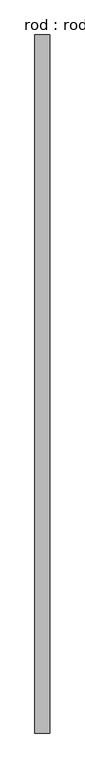
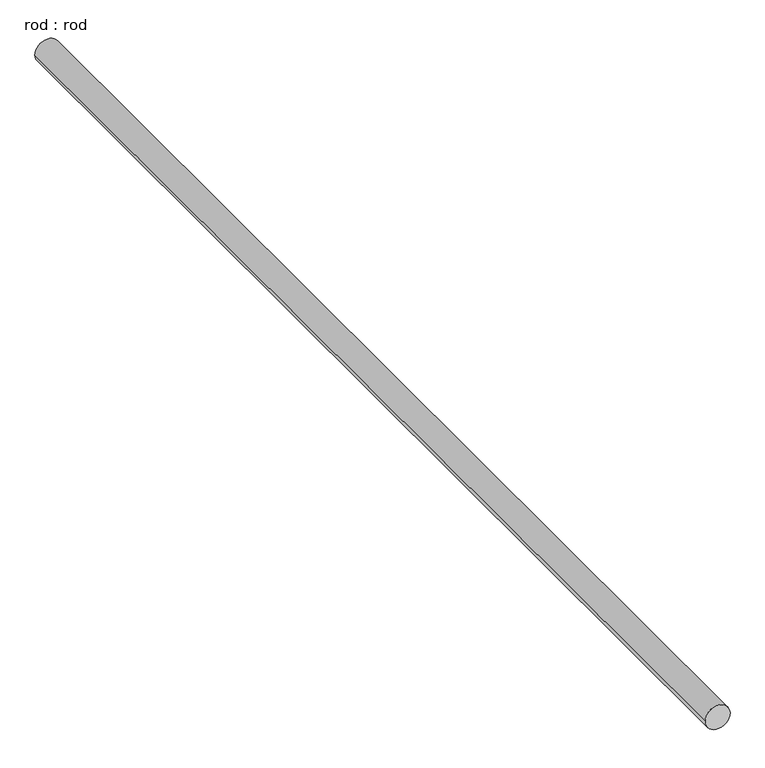
"""IFC4 building model written with IfcOpenShell, lengths in millimetres: proxy geometry, rod : rod."""

import ifcopenshell
import ifcopenshell.guid

model = None  # the IFC model being written
_history = None  # IfcOwnerHistory: only IFC2X3 demands one
_inside = {}  # id of a spatial element -> (the spatial element, [elements in it])
_under = {}  # id of a project, library or spatial element -> (it, [spatial elements below it])
_declared = {}  # id of a project -> (the project, [libraries it declares])
_typed = {}  # id of a type object -> (the type object, [elements of that type])
_made_of = {}  # id of a material, layer set ... -> (it, [elements and type objects made of it])


def new_model(schema):
    """Start an empty IFC model of exactly this schema.

    Asked for "IFC4X3", IfcOpenShell would pick the latest addendum, in which some entities
    have other attributes; the version numbers below select the first issue.
    IFC2X3 requires an IfcOwnerHistory on every rooted entity: one is made here for all.
    """
    global model, _history
    if schema == "IFC4X3":
        model = ifcopenshell.file(schema_version=(4, 3, 0, 0))
    else:
        model = ifcopenshell.file(schema=schema)
    _inside.clear()
    _under.clear()
    _declared.clear()
    _typed.clear()
    _made_of.clear()
    _history = None
    if model.schema == "IFC2X3":
        org = make("IfcOrganization", Name="unknown")
        user = make(
            "IfcPersonAndOrganization",
            ThePerson=make("IfcPerson", FamilyName="unknown"),
            TheOrganization=org,
        )
        app = make(
            "IfcApplication",
            ApplicationDeveloper=org,
            Version="unknown",
            ApplicationFullName="unknown",
            ApplicationIdentifier="unknown",
        )
        _history = make(
            "IfcOwnerHistory",
            OwningUser=user,
            OwningApplication=app,
            ChangeAction="ADDED",
            CreationDate=0,
        )
    return model


def make(cls, **values):
    """One entity of the class cls with the attributes given. An attribute that is None is left unset."""
    return model.create_entity(
        cls, **{name: value for name, value in values.items() if value is not None}
    )


def rooted(cls, **values):
    """An entity with a GlobalId (a new one), such as an element, a storey or a relation."""
    return make(cls, GlobalId=ifcopenshell.guid.new(), OwnerHistory=_history, **values)


def si_unit(unit_type, name, prefix=None):
    """IfcSIUnit, for example si_unit("LENGTHUNIT", "METRE", prefix="MILLI")."""
    return make("IfcSIUnit", UnitType=unit_type, Prefix=prefix, Name=name)


def assignment(units):
    """IfcUnitAssignment: the units of a project."""
    return None if units is None else make("IfcUnitAssignment", Units=units)


def point(xyz):
    """IfcCartesianPoint."""
    return None if xyz is None else make("IfcCartesianPoint", Coordinates=xyz)


def direction(xyz):
    """IfcDirection."""
    return None if xyz is None else make("IfcDirection", DirectionRatios=xyz)


def frame(location, z_axis=None, x_axis=None):
    """IfcAxis2Placement3D, a coordinate frame: its origin and axes. An axis left out is left unset."""
    return make(
        "IfcAxis2Placement3D",
        Location=point(location),
        Axis=direction(z_axis),
        RefDirection=direction(x_axis),
    )


def frame_2d(location, x_axis=None):
    """IfcAxis2Placement2D, a coordinate frame in the plane: its origin and x axis."""
    return make(
        "IfcAxis2Placement2D", Location=point(location), RefDirection=direction(x_axis)
    )


def origin():
    """The frame at (0, 0, 0) with its axes left unset."""
    return frame((0.0, 0.0, 0.0))


def place(relative_to, where):
    """IfcLocalPlacement: puts the frame where relative to a parent placement (None: the world)."""
    return make(
        "IfcLocalPlacement", PlacementRelTo=relative_to, RelativePlacement=where
    )


def context(
    kind, dimensions, precision=None, world=None, true_north=None, identifier=None
):
    """IfcGeometricRepresentationContext, for example the 3D "Model" context."""
    return make(
        "IfcGeometricRepresentationContext",
        ContextIdentifier=identifier,
        ContextType=kind,
        CoordinateSpaceDimension=dimensions,
        Precision=precision,
        WorldCoordinateSystem=world,
        TrueNorth=true_north,
    )


def project(units=None, contexts=None):
    """IfcProject with its units and contexts."""
    return rooted(
        "IfcProject",
        Name="project",
        RepresentationContexts=contexts,
        UnitsInContext=assignment(units),
    )


def spatial(cls, under=None, at=None, **own):
    """A site, building, storey or space (cls), placed at a placement, below another one or the project."""
    s = rooted(cls, ObjectPlacement=at, **own)
    if under is not None:
        _under.setdefault(under.id(), (under, []))[1].append(s)
    return s


def circle_curve(where, radius):
    """IfcCircle in the frame where."""
    return make("IfcCircle", Position=where, Radius=radius)


def trimmed(basis, trim1, trim2, sense, master):
    """IfcTrimmedCurve: the piece of a basis curve between two trims."""
    return make(
        "IfcTrimmedCurve",
        BasisCurve=basis,
        Trim1=trim1,
        Trim2=trim2,
        SenseAgreement=sense,
        MasterRepresentation=master,
    )


def segment(curve, same_sense, transition):
    """IfcCompositeCurveSegment."""
    return make(
        "IfcCompositeCurveSegment",
        Transition=transition,
        SameSense=same_sense,
        ParentCurve=curve,
    )


def composite_curve(segments, self_intersect=None):
    """IfcCompositeCurve: segments joined end to end."""
    return make("IfcCompositeCurve", Segments=segments, SelfIntersect=self_intersect)


def outline(outer, holes=None, kind="AREA"):
    """IfcArbitraryClosedProfileDef: a profile drawn as a closed curve; with holes, ...WithVoids."""
    if holes is None:
        return make("IfcArbitraryClosedProfileDef", ProfileType=kind, OuterCurve=outer)
    return make(
        "IfcArbitraryProfileDefWithVoids",
        ProfileType=kind,
        OuterCurve=outer,
        InnerCurves=holes,
    )


def extrude(swept, where, along, depth):
    """IfcExtrudedAreaSolid: the profile swept, set in the frame where, extruded along a direction by depth."""
    return make(
        "IfcExtrudedAreaSolid",
        SweptArea=swept,
        Position=where,
        ExtrudedDirection=direction(along),
        Depth=depth,
    )


def shape(context_of_items, identifier, shape_type, items):
    """IfcShapeRepresentation: the items that make up one representation, for example the "Body"."""
    return make(
        "IfcShapeRepresentation",
        ContextOfItems=context_of_items,
        RepresentationIdentifier=identifier,
        RepresentationType=shape_type,
        Items=items,
    )


def source(mapping_origin, context_of_items, identifier, shape_type, items):
    """IfcRepresentationMap: a shape defined once, which mapped items show again and again."""
    return make(
        "IfcRepresentationMap",
        MappingOrigin=mapping_origin,
        MappedRepresentation=shape(context_of_items, identifier, shape_type, items),
    )


def transform(
    local_origin,
    x_axis=None,
    y_axis=None,
    z_axis=None,
    scale=None,
    scale2=None,
    scale3=None,
    uniform=True,
):
    """IfcCartesianTransformationOperator3D, or its non-uniform kind. x_axis, y_axis, z_axis: its Axis1, 2, 3."""
    if uniform:
        return make(
            "IfcCartesianTransformationOperator3D",
            Axis1=direction(x_axis),
            Axis2=direction(y_axis),
            LocalOrigin=point(local_origin),
            Scale=scale,
            Axis3=direction(z_axis),
        )
    return make(
        "IfcCartesianTransformationOperator3DnonUniform",
        Axis1=direction(x_axis),
        Axis2=direction(y_axis),
        LocalOrigin=point(local_origin),
        Scale=scale,
        Axis3=direction(z_axis),
        Scale2=scale2,
        Scale3=scale3,
    )


def mapped(mapping_source, mapping_target):
    """IfcMappedItem: shows the shape of a source again, moved by a transform."""
    return make(
        "IfcMappedItem", MappingSource=mapping_source, MappingTarget=mapping_target
    )


def made_of(thing, what):
    """Note that an element or type object is made of a material, layer set ...; save() writes the relation."""
    if what is not None:
        _made_of.setdefault(what.id(), (what, []))[1].append(thing)
    return thing


def element(
    cls,
    number,
    at=None,
    inside=None,
    cuts=None,
    type_object=None,
    material=None,
    context=None,
    identifier="Body",
    shape_type=None,
    held_by="IfcProductDefinitionShape",
    body=None,
    shapes=None,
    **own,
):
    """One element of the class cls, such as IfcWall. Its Tag is "e" and its number.

    at: its placement. inside: the storey or other place that contains it. cuts: it is an
    opening in that element (IfcRelVoidsElement). A single representation is given by context,
    identifier, shape_type and body (its items); several are given by shapes. held_by: the class
    of the entity that holds the representations. save() writes the other relations.
    """
    e = rooted(cls, Tag="e%d" % number, ObjectPlacement=at, **own)
    if body is not None:
        shapes = [shape(context, identifier, shape_type, body)]
    if shapes is not None:
        e.Representation = make(held_by, Representations=shapes)
    if inside is not None:
        _inside.setdefault(inside.id(), (inside, []))[1].append(e)
    if cuts is not None:
        rooted(
            "IfcRelVoidsElement", RelatingBuildingElement=cuts, RelatedOpeningElement=e
        )
    if type_object is not None:
        _typed.setdefault(type_object.id(), (type_object, []))[1].append(e)
    return made_of(e, material)


def aggregate(whole, parts):
    """IfcRelAggregates: a whole, such as a stair, and the parts it consists of."""
    return rooted("IfcRelAggregates", RelatingObject=whole, RelatedObjects=parts)


def save(model, path):
    """Write the relations noted so far, then the file.

    IfcRelAggregates (storeys below a building ...), IfcRelContainedInSpatialStructure (elements
    in a storey), IfcRelDefinesByType, IfcRelAssociatesMaterial and IfcRelDeclares: one each for
    every whole, place, type object, material and project.
    """
    for whole, parts in _under.values():
        aggregate(whole, parts)
    for where, things in _inside.values():
        rooted(
            "IfcRelContainedInSpatialStructure",
            RelatedElements=things,
            RelatingStructure=where,
        )
    for kind, things in _typed.values():
        rooted("IfcRelDefinesByType", RelatedObjects=things, RelatingType=kind)
    for what, things in _made_of.values():
        rooted("IfcRelAssociatesMaterial", RelatedObjects=things, RelatingMaterial=what)
    for by, libraries in _declared.values():
        rooted("IfcRelDeclares", RelatingContext=by, RelatedDefinitions=libraries)
    model.write(path)


def rod_rod_b9634de2(model_context):
    return source(origin(), model_context, "Body", "SweptSolid", [
        extrude(outline(composite_curve([segment(trimmed(circle_curve(frame_2d((0.0108462, 0.0)), 200.0), [point((0.0108462, 200.0))], [point((0.0108462, -200.0))], False, "CARTESIAN"), True, "CONTINUOUS"), segment(trimmed(circle_curve(frame_2d((0.0108462, 0.0)), 200.0), [point((0.0108462, -200.0))], [point((0.0108462, 200.0))], False, "CARTESIAN"), True, "CONTINUOUS")], self_intersect=False)), frame((0.0, -5191.2683853, 0.0), z_axis=(0.0, 1.0, 0.0), x_axis=(0.0, 0.0, 1.0)), (0.0, 0.0, 1.0), 18567.9940014),
    ])


if __name__ == "__main__":
    model = new_model("IFC4")
    model_context = context("Model", 3, world=origin())
    ifc_project = project(units=[si_unit("LENGTHUNIT", "METRE", prefix="MILLI")], contexts=[model_context])
    site = spatial("IfcSite", under=ifc_project)
    building = spatial("IfcBuilding", under=site)
    placement = place(None, origin())
    rod_rod_shape = rod_rod_b9634de2(model_context)
    element("IfcBuildingElementProxy", 1, Name="rod : rod", ObjectType="rod : rod", at=placement, inside=building, context=model_context, shape_type="MappedRepresentation", body=[
        mapped(rod_rod_shape, transform((0.0, 0.0, 0.0), x_axis=(1.0, 0.0, 0.0), y_axis=(0.0, 1.0, 0.0), z_axis=(0.0, 0.0, 1.0))),
    ])
    save(model, "model.ifc")

# Revit data of these elements
# Type "rod : rod"
#   Default Elevation = 0
